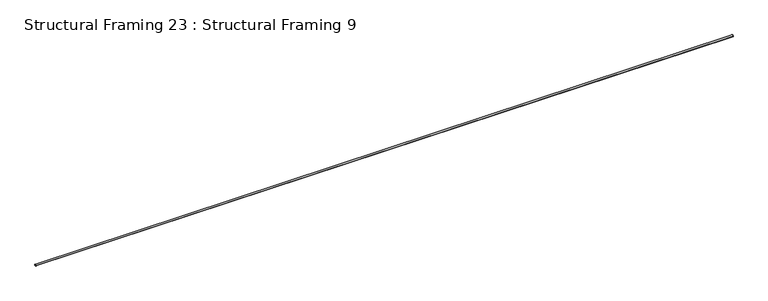
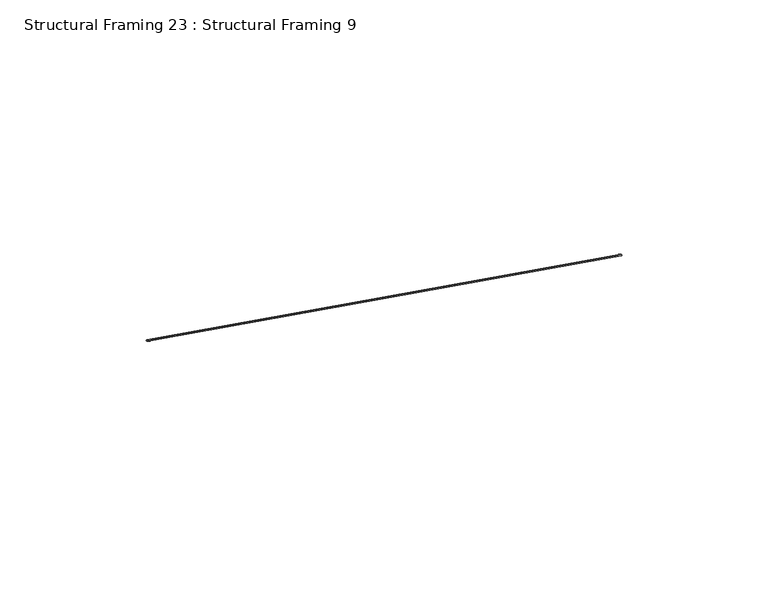
"""IFC4 building model written with IfcOpenShell, lengths in millimetres: beam geometry, Structural Framing 23 : Structural Framing 9."""

from ifc_helpers import new_model, si_unit, point, frame, origin, origin_2d, place, context, project, spatial, circle_curve, trimmed, segment, composite_curve, outline, extrude, source, transform, mapped, element, save


def structural_framing_23_structural_framing_9_4030a1bf(model_context):
    return source(origin(), model_context, "Body", "SweptSolid", [
        extrude(outline(composite_curve([segment(trimmed(circle_curve(origin_2d(), 6.35), [point((0.0, -6.35))], [point((0.0, 6.3499999))], False, "CARTESIAN"), True, "CONTINUOUS"), segment(trimmed(circle_curve(origin_2d(), 6.35), [point((0.0, 6.3499999))], [point((0.0, -6.35))], False, "CARTESIAN"), True, "CONTINUOUS")], self_intersect=False)), frame((28306.0390052, 11682.7351788, 2966.1078019), z_axis=(-0.8890536510975664, -0.2930783517672797, 0.35169402212073736), x_axis=(0.0, -0.7682212795973776, -0.6401843996644778)), (0.0, 0.0, 1.0), 5574.8064179),
    ])


if __name__ == "__main__":
    model = new_model("IFC4")
    model_context = context("Model", 3, world=origin())
    ifc_project = project(units=[si_unit("LENGTHUNIT", "METRE", prefix="MILLI")], contexts=[model_context])
    site = spatial("IfcSite", under=ifc_project)
    building = spatial("IfcBuilding", under=site)
    placement = place(None, origin())
    structural_framing_23_structural_framing_9_shape = structural_framing_23_structural_framing_9_4030a1bf(model_context)
    element("IfcBeam", 1, ObjectType="Structural Framing 23 : Structural Framing 9", at=placement, inside=building, context=model_context, shape_type="MappedRepresentation", body=[
        mapped(structural_framing_23_structural_framing_9_shape, transform((0.0, 0.0, 0.0), x_axis=(1.0, 0.0, 0.0), y_axis=(0.0, 1.0, 0.0), z_axis=(0.0, 0.0, 1.0))),
    ])
    save(model, "model.ifc")

# Revit data of these elements
# Type "Structural Framing 23 : Structural Framing 9"
#   Structural Material [instance default] = EXISTING LATERAL BRACING (1/4" CABLE)
# Element 1 (IfcBeam, "Structural Framing 23 : Structural Framing 9")
#   Materials on its faces: "EXISTING LATERAL BRACING (1/4\" CABLE)"
# Materials
#   "EXISTING LATERAL BRACING (1/4\" CABLE)": class "Generic", colour RGB 120 120 120, transparency 0, Cost = 0
